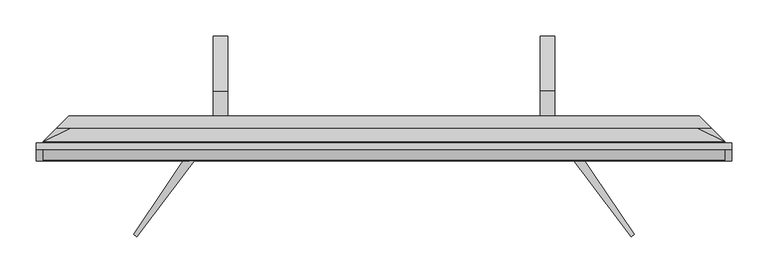
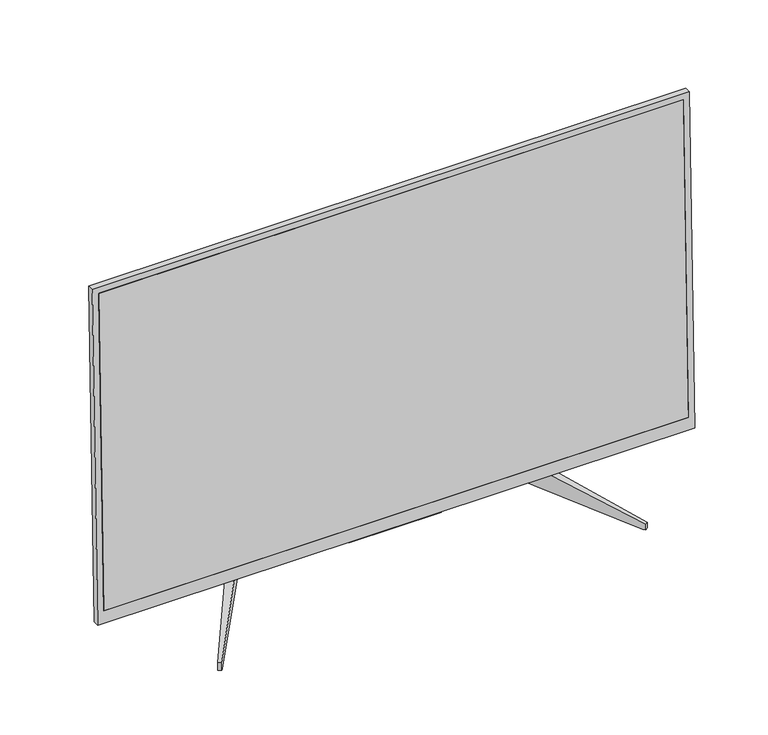
"""IFC4 building model written with IfcOpenShell, lengths in millimetres: proxy geometry, Electronics_Visual-TVs_Sony-Professional_FW-43BZ35F-43in-BRAVIA-4K-HDR-Professional-Display : FW-43BZ35F."""

from ifc_helpers import new_model, si_unit, point, frame, frame_2d, origin, place, context, project, spatial, polyline, circle_curve, trimmed, segment, composite_curve, outline, extrude, faceted_brep, source, transform, mapped, element, save
from ifc_brep_helpers import plane_surface, revolved_surface, advanced_brep


def communication_devices_8732f4fb(model_context):
    return source(origin(), model_context, "Body", "SolidModel", [
        extrude(outline(polyline([(0.0, -10.0000001), (0.0, 0.0), (944.8, 0.0), (944.8, -10.0000001), (0.0, -10.0000001)])), frame((472.4, -33.3449697, 83.2957538), z_axis=(0.0, 0.02617694830787593, 0.9996573249755573), x_axis=(-1.0, 0.0, 0.0)), (0.0, 0.0, 1.0), 534.3),
        faceted_brep([(482.4, -33.9, 62.1), (482.4, -23.8965721, 62.1), (482.4, -9.0936706, 627.4), (482.4, -19.0970985, 627.4), (-482.4, -33.9, 62.1), (-482.4, -19.0970985, 627.4), (-482.4, -9.0936706, 627.4), (-482.4, -23.8965721, 62.1), (-472.4, -23.3483964, 83.0339843), (472.4, -23.3483964, 83.0339843), (472.4, -9.3620529, 617.150893), (-472.4, -9.3620529, 617.150893), (472.4, -33.3449697, 83.2957538), (-472.4, -33.3449697, 83.2957538), (-472.4, -19.3586262, 617.4126625), (472.4, -19.3586262, 617.4126625)], [[[0, 1, 2, 3]], [[4, 5, 6, 7]], [[1, 0, 4, 7]], [[2, 1, 7, 6], [8, 9, 10, 11]], [[0, 3, 5, 4], [12, 13, 14, 15]], [[8, 13, 12, 9]], [[9, 12, 15, 10]], [[10, 15, 14, 11]], [[13, 8, 11, 14]], [[3, 2, 6, 5]]]),
        faceted_brep([(-236.5680468, 139.3, 32.6847301), (-216.5680468, 139.3, 32.6847301), (-216.5680468, 130.7, 0.0), (-236.5680468, 130.7, 0.0), (-216.5680468, 28.1, 37.1705579), (-236.5680468, 28.1, 37.1705579), (-236.5680468, 120.1003592, 0.0), (-216.5680468, 120.1003592, 0.0), (-236.5680468, 62.670602, 62.1), (-216.5680468, 62.670602, 62.1), (-339.9507568, -135.8671682, 0.0), (-347.1652982, -135.8671682, 0.0), (-216.5680468, 28.1, 62.1), (-236.5680468, 28.1, 62.1), (-258.0876491, -3.8041224, 62.1), (-246.471337, -11.6394239, 62.1), (-342.5339087, -139.3, 0.0), (-347.1652982, -135.8671682, 13.3980759), (-342.5339087, -139.3, 13.3197763)], [[[0, 1, 2, 3]], [[4, 5, 6, 7]], [[1, 0, 8, 9]], [[5, 4, 10, 11]], [[12, 9, 8, 13, 14, 15]], [[16, 11, 10]], [[6, 3, 2, 7]], [[13, 5, 11, 17, 14]], [[11, 16, 18, 17]], [[16, 10, 4, 12, 15, 18]], [[9, 12, 4, 7, 2, 1]], [[13, 8, 0, 3, 6, 5]], [[15, 14, 17, 18]]]),
        faceted_brep([(236.5680468, 28.1, 62.1), (236.5680468, 62.670602, 62.1), (216.5680468, 62.670602, 62.1), (216.5680468, 28.1, 62.1), (238.7109742, -1.3264334, 62.1), (250.8799901, 6.8816715, 62.1), (347.1652982, -135.8671682, 0.0), (342.5339087, -139.3, 0.0), (339.9507568, -135.8671682, 0.0), (216.5680468, 120.1003592, 0.0), (216.5680468, 130.7, 0.0), (236.5680468, 130.7, 0.0), (236.5680468, 120.1003592, 0.0), (236.5680468, 28.1, 37.1705579), (347.1652982, -135.8671682, 9.4573919), (342.5339087, -139.3, 9.3790923), (216.5680468, 28.1, 37.1705579), (216.5680468, 139.3, 32.6847301), (236.5680468, 139.3, 32.6847301)], [[[0, 1, 2, 3, 4, 5]], [[6, 7, 8]], [[9, 10, 11, 12]], [[13, 0, 5, 14, 6]], [[7, 6, 14, 15]], [[8, 7, 15, 4, 3, 16]], [[3, 2, 17, 10, 9, 16]], [[1, 0, 13, 12, 11, 18]], [[17, 18, 11, 10]], [[13, 16, 9, 12]], [[18, 17, 2, 1]], [[16, 13, 6, 8]], [[5, 4, 15, 14]]]),
        extrude(outline(composite_curve([segment(trimmed(circle_curve(frame_2d((64.9596066, 9.5619733)), 10.0), [point((64.9596066, 19.5619733))], [point((74.9596066, 9.5619733))], False, "CARTESIAN"), True, "CONTINUOUS"), segment(polyline([(74.9596066, 9.5619733), (74.9596066, -30.5494977), (-74.9596066, -30.5494977), (-74.9596066, 9.5619733)]), True, "CONTINUOUS"), segment(trimmed(circle_curve(frame_2d((-64.9596066, 9.5619733)), 10.0), [point((-74.9596066, 9.5619733))], [point((-64.9596066, 19.5619733))], False, "CARTESIAN"), True, "CONTINUOUS"), segment(polyline([(-64.9596066, 19.5619733), (64.9596066, 19.5619733)]), True, "CONTINUOUS")], self_intersect=False)), frame((0.0, 0.0, 58.1), z_axis=(0.0, 0.0, 1.0), x_axis=(1.0, 0.0, 0.0)), (0.0, 0.0, 1.0), 4.0),
        faceted_brep([(-472.4, -7.1375823, 617.1811048), (-472.4, -9.3612618, 617.1811048), (472.4, -9.3612618, 617.1811048), (472.4, -7.1375823, 617.1811048), (471.9010922, -6.8942487, 617.1811048), (-471.9010922, -6.8942487, 617.1811048), (435.1742293, 11.0186392, 526.6060744), (472.4, -7.1375823, 526.6060744), (472.4, -11.7330524, 526.6060744), (-472.4, -11.7330524, 526.6060744), (-472.4, -7.1375823, 526.6060744), (-435.1742293, 11.0186392, 526.6060744)], [[[0, 1, 2, 3, 4, 5]], [[6, 7, 8, 9, 10, 11]], [[0, 10, 9, 1]], [[7, 3, 2, 8]], [[2, 1, 9, 8]], [[11, 10, 0, 5]], [[7, 6, 4, 3]], [[5, 4, 6, 11]]]),
        advanced_brep(
        [(-472.4, -7.1375823, 526.6060744), (-472.4, -11.7330524, 526.6060744), (472.4, -11.7330524, 526.6060744), (472.4, -7.1375823, 526.6060744), (454.2437785, 11.0186392, 526.6060744), (-454.2437785, 11.0186392, 526.6060744), (-472.4, -7.1375823, 170.6631269), (-437.1624177, 28.1, 170.6631269), (437.1624177, 28.1, 170.6631269), (472.4, -7.1375823, 170.6631269), (472.4, -21.0537465, 170.6631269), (-472.4, -21.0537465, 170.6631269), (437.1624177, 28.1, 523.5941696), (-437.1624177, 28.1, 172.1), (-322.3011917, 28.1, 172.1), (-322.3011917, 28.1, 473.9795749), (-437.1624177, 28.1, 473.9795749), (-437.1624177, 28.1, 523.5941696), (212.1, 28.1, 266.75), (160.2, 28.1, 266.75), (160.2, 28.1, 179.75), (212.1, 28.1, 179.75), (-147.0, 28.1, 343.2), (-293.6, 28.1, 343.2), (-293.6, 28.1, 253.0), (-147.0, 28.1, 253.0), (100.0, 28.1, 326.3), (100.0, 28.1, 320.3), (-100.0, 28.1, 326.3), (-100.0, 28.1, 320.3), (-452.5963815, 12.6660362, 473.9795749), (-452.5963815, 12.6660362, 172.1), (-322.3011917, 12.6660362, 473.9795749), (-322.3011917, 12.6660362, 172.1), (212.1, 25.6497626, 266.75), (212.1, 25.6497626, 179.75), (160.2, 25.6497626, 179.75), (160.2, 25.6497626, 266.75), (-147.0, 25.6497626, 343.2), (-147.0, 25.6497626, 253.0), (-293.6, 25.6497626, 253.0), (-293.6, 25.6497626, 343.2), (100.0, 21.959368, 326.3), (100.0, 21.959368, 320.3), (-100.0, 21.959368, 326.3), (-100.0, 21.959368, 320.3)],
        [
            (0, 1),
            (1, 2),
            (2, 3),
            (3, 4),
            (4, 5),
            (5, 0),
            (6, 7),
            (7, 8),
            (8, 9),
            (9, 10),
            (10, 11),
            (11, 6),
            (0, 6),
            (11, 1),
            (9, 3),
            (2, 10),
            (8, 12),
            (12, 4),
            (7, 13),
            (13, 14),
            (14, 15),
            (15, 16),
            (16, 17),
            (17, 12),
            (18, 19),
            (19, 20),
            (20, 21),
            (21, 18),
            (22, 23),
            (23, 24),
            (24, 25),
            (25, 22),
            (26, 27, circle_curve(frame((100.0, 28.1, 323.3), z_axis=(0.0, -1.0, 0.0), x_axis=(0.0, 0.0, -1.0)), 3.0)),
            (27, 26, circle_curve(frame((100.0, 28.1, 323.3), z_axis=(0.0, -1.0, 0.0), x_axis=(0.0, 0.0, -1.0)), 3.0)),
            (28, 29, circle_curve(frame((-100.0, 28.1, 323.3), z_axis=(0.0, -1.0, 0.0), x_axis=(0.0, 0.0, -1.0)), 3.0)),
            (29, 28, circle_curve(frame((-100.0, 28.1, 323.3), z_axis=(0.0, -1.0, 0.0), x_axis=(0.0, 0.0, -1.0)), 3.0)),
            (5, 17),
            (16, 30),
            (30, 31),
            (31, 13),
            (32, 33),
            (33, 31),
            (30, 32),
            (32, 15),
            (14, 33),
            (34, 35),
            (35, 36),
            (36, 37),
            (37, 34),
            (38, 39),
            (39, 40),
            (40, 41),
            (41, 38),
            (37, 19),
            (18, 34),
            (36, 20),
            (35, 21),
            (41, 23),
            (22, 38),
            (40, 24),
            (39, 25),
            (42, 43, circle_curve(frame((100.0, 21.959368, 323.3), z_axis=(0.0, 1.0, 0.0), x_axis=(0.0, 0.0, -1.0)), 3.0)),
            (43, 42, circle_curve(frame((100.0, 21.959368, 323.3), z_axis=(0.0, 1.0, 0.0), x_axis=(0.0, 0.0, -1.0)), 3.0)),
            (44, 45, circle_curve(frame((-100.0, 21.959368, 323.3), z_axis=(0.0, 1.0, 0.0), x_axis=(0.0, 0.0, -1.0)), 3.0)),
            (45, 44, circle_curve(frame((-100.0, 21.959368, 323.3), z_axis=(0.0, 1.0, 0.0), x_axis=(0.0, 0.0, -1.0)), 3.0)),
            (43, 27),
            (26, 42),
            (45, 29),
            (28, 44),
        ],
        [
            plane_surface(frame((-472.4, -7.1375823, 526.6060744), z_axis=(0.0, 0.0, 1.0), x_axis=(0.0, -1.0, 0.0))),
            plane_surface(frame((-472.4, -7.1375823, 170.6631269), z_axis=(0.0, 0.0, -1.0), x_axis=(0.0, 1.0, 0.0))),
            plane_surface(frame((-472.4, -7.1375823, 526.6060744), z_axis=(-1.0, 0.0, 0.0), x_axis=(0.0, 0.0, -1.0))),
            plane_surface(frame((472.4, -27.5708403, 526.6060744), z_axis=(1.0, 0.0, 0.0), x_axis=(0.0, 0.0, -1.0))),
            plane_surface(frame((472.4, -7.1375823, 526.6060744), z_axis=(0.707106781186642, 0.7071067811864531, 0.0), x_axis=(0.0, 0.0, -1.0))),
            plane_surface(frame((437.1624177, 28.1, 526.6060744), z_axis=(0.0, 1.0, 0.0), x_axis=(0.0, 0.0, -1.0))),
            plane_surface(frame((-437.1624177, 28.1, 526.6060744), z_axis=(-0.7071067811865435, 0.7071067811865518, 0.0), x_axis=(0.0, 0.0, -1.0))),
            plane_surface(frame((625.5732366, -23.8965721, 62.1), z_axis=(0.0, -0.9996573249755574, 0.026176948307870252), x_axis=(-1.0, 0.0, 0.0))),
            plane_surface(frame((587.9862131, 11.0186392, 526.6060744), z_axis=(0.0, 0.17364817766693166, 0.9848077530122079), x_axis=(-1.0, 0.0, 0.0))),
            plane_surface(frame((-322.3011917, 12.6660362, 172.1), z_axis=(0.0, 1.0, 0.0), x_axis=(1.0, 0.0, 0.0))),
            plane_surface(frame((-322.3011917, 12.6660362, 172.1), z_axis=(-1.0, 0.0, 0.0), x_axis=(0.0, 1.0, 0.0))),
            plane_surface(frame((-322.3011917, 12.6660362, 473.9795749), z_axis=(0.0, 0.0, -1.0), x_axis=(0.0, 1.0, 0.0))),
            plane_surface(frame((-464.2088994, 12.6660362, 172.1), z_axis=(0.0, 0.0, 1.0), x_axis=(0.0, 1.0, 0.0))),
            plane_surface(frame((194.45, 25.6497626, 266.75), z_axis=(0.0, 1.0, 0.0), x_axis=(-1.0, 0.0, 0.0))),
            plane_surface(frame((212.1, 25.6497626, 266.75), z_axis=(0.0, 0.0, -1.0), x_axis=(0.0, 1.0, 0.0))),
            plane_surface(frame((160.2, 25.6497626, 266.75), z_axis=(1.0, 0.0, 0.0), x_axis=(0.0, 1.0, 0.0))),
            plane_surface(frame((160.2, 25.6497626, 179.75), z_axis=(0.0, 0.0, 1.0), x_axis=(0.0, 1.0, 0.0))),
            plane_surface(frame((212.1, 25.6497626, 179.75), z_axis=(-1.0, 0.0, 0.0), x_axis=(0.0, 1.0, 0.0))),
            plane_surface(frame((-147.0, 25.6497626, 343.2), z_axis=(0.0, 0.0, -1.0), x_axis=(0.0, 1.0, 0.0))),
            plane_surface(frame((-293.6, 25.6497626, 343.2), z_axis=(1.0, 0.0, 0.0), x_axis=(0.0, 1.0, 0.0))),
            plane_surface(frame((-293.6, 25.6497626, 253.0), z_axis=(0.0, 0.0, 1.0), x_axis=(0.0, 1.0, 0.0))),
            plane_surface(frame((-147.0, 25.6497626, 253.0), z_axis=(-1.0, 0.0, 0.0), x_axis=(0.0, 1.0, 0.0))),
            plane_surface(frame((100.0, 21.959368, 320.3), z_axis=(0.0, 1.0, 0.0), x_axis=(1.0, 0.0, 0.0))),
            revolved_surface(polyline([(100.0, 21.959368, 320.3), (100.0, 28.1, 320.3)]), (100.0, 36.8651248, 323.3), (0.0, -1.0, 0.0)),
            revolved_surface(polyline([(-100.0, 21.959368, 320.3), (-100.0, 28.1, 320.3)]), (-100.0, 36.8651248, 323.3), (0.0, -1.0, 0.0)),
        ],
        [
            (0, [[1, 2, 3, 4, 5, 6]]),
            (1, [[7, 8, 9, 10, 11, 12]]),
            (2, [[13, -12, 14, -1]]),
            (3, [[15, -3, 16, -10]]),
            (4, [[-9, 17, 18, -4, -15]]),
            (5, [[-8, 19, 20, 21, 22, 23, 24, -17], [25, 26, 27, 28], [29, 30, 31, 32], [33, 34], [35, 36]]),
            (6, [[-7, -13, -6, 37, -23, 38, 39, 40, -19]]),
            (7, [[-2, -14, -11, -16]]),
            (8, [[-5, -18, -24, -37]]),
            (9, [[41, 42, -39, 43]]),
            (10, [[-41, 44, -21, 45]]),
            (11, [[-43, -38, -22, -44]]),
            (12, [[-42, -45, -20, -40]]),
            (13, [[46, 47, 48, 49]]),
            (13, [[50, 51, 52, 53]]),
            (14, [[-49, 54, -25, 55]]),
            (15, [[-48, 56, -26, -54]]),
            (16, [[-47, 57, -27, -56]]),
            (17, [[-46, -55, -28, -57]]),
            (18, [[-53, 58, -29, 59]]),
            (19, [[-52, 60, -30, -58]]),
            (20, [[-51, 61, -31, -60]]),
            (21, [[-50, -59, -32, -61]]),
            (22, [[62, 63]]),
            (22, [[64, 65]]),
            (23, [[-63, 66, -33, 67]]),
            (23, [[-62, -67, -34, -66]]),
            (24, [[-65, 68, -35, 69]]),
            (24, [[-64, -69, -36, -68]]),
        ],
    ),
        advanced_brep(
        [(437.1624177, 28.1, 170.6631269), (-437.1624177, 28.1, 170.6631269), (-472.4, -7.1375823, 170.6631269), (-472.4, -21.0537465, 170.6631269), (472.4, -21.0537465, 170.6631269), (472.4, -7.1375823, 170.6631269), (437.1624177, 28.1, 62.1), (472.4, -7.1375823, 62.1), (472.4, -23.8965721, 62.1), (-472.4, -23.8965721, 62.1), (-472.4, -7.1375823, 62.1), (-437.1624177, 28.1, 62.1), (100.0, 28.1, 126.3), (100.0, 28.1, 120.3), (-100.0, 28.1, 126.3), (-100.0, 28.1, 120.3), (100.0, 21.959368, 126.3), (100.0, 21.959368, 120.3), (-100.0, 21.959368, 126.3), (-100.0, 21.959368, 120.3)],
        [
            (0, 1),
            (1, 2),
            (2, 3),
            (3, 4),
            (4, 5),
            (5, 0),
            (6, 7),
            (7, 8),
            (8, 9),
            (9, 10),
            (10, 11),
            (11, 6),
            (0, 6),
            (11, 1),
            (12, 13, circle_curve(frame((100.0, 28.1, 123.3), z_axis=(0.0, -1.0, 0.0), x_axis=(0.0, 0.0, -1.0)), 3.0)),
            (13, 12, circle_curve(frame((100.0, 28.1, 123.3), z_axis=(0.0, -1.0, 0.0), x_axis=(0.0, 0.0, -1.0)), 3.0)),
            (14, 15, circle_curve(frame((-100.0, 28.1, 123.3), z_axis=(0.0, -1.0, 0.0), x_axis=(0.0, 0.0, -1.0)), 3.0)),
            (15, 14, circle_curve(frame((-100.0, 28.1, 123.3), z_axis=(0.0, -1.0, 0.0), x_axis=(0.0, 0.0, -1.0)), 3.0)),
            (2, 10),
            (9, 3),
            (7, 5),
            (4, 8),
            (16, 17, circle_curve(frame((100.0, 21.959368, 123.3), z_axis=(0.0, 1.0, 0.0), x_axis=(0.0, 0.0, -1.0)), 3.0)),
            (17, 16, circle_curve(frame((100.0, 21.959368, 123.3), z_axis=(0.0, 1.0, 0.0), x_axis=(0.0, 0.0, -1.0)), 3.0)),
            (18, 19, circle_curve(frame((-100.0, 21.959368, 123.3), z_axis=(0.0, 1.0, 0.0), x_axis=(0.0, 0.0, -1.0)), 3.0)),
            (19, 18, circle_curve(frame((-100.0, 21.959368, 123.3), z_axis=(0.0, 1.0, 0.0), x_axis=(0.0, 0.0, -1.0)), 3.0)),
            (17, 13),
            (12, 16),
            (19, 15),
            (14, 18),
        ],
        [
            plane_surface(frame((-437.1624177, 28.1, 170.6631269), z_axis=(0.0, 0.0, 1.0), x_axis=(-1.0, 0.0, 0.0))),
            plane_surface(frame((-437.1624177, 28.1, 62.1), z_axis=(0.0, 0.0, -1.0), x_axis=(1.0, 0.0, 0.0))),
            plane_surface(frame((437.1624177, 28.1, 170.6631269), z_axis=(0.0, 1.0, 0.0), x_axis=(0.0, 0.0, -1.0))),
            plane_surface(frame((-472.4, -7.1375823, 170.6631269), z_axis=(-1.0, 0.0, 0.0), x_axis=(0.0, 0.0, -1.0))),
            plane_surface(frame((472.4, -27.5708403, 170.6631269), z_axis=(1.0, 0.0, 0.0), x_axis=(0.0, 0.0, -1.0))),
            plane_surface(frame((-437.1624177, 28.1, 170.6631269), z_axis=(-0.7071067811865488, 0.7071067811865462, 0.0), x_axis=(0.0, 0.0, -1.0))),
            plane_surface(frame((472.4, -7.1375823, 170.6631269), z_axis=(0.7071067811866403, 0.7071067811864549, 0.0), x_axis=(0.0, 0.0, -1.0))),
            plane_surface(frame((625.5732366, -23.8965721, 62.1), z_axis=(0.0, -0.9996573249755574, 0.026176948307870252), x_axis=(-1.0, 0.0, 0.0))),
            plane_surface(frame((100.0, 21.959368, 320.3), z_axis=(0.0, 1.0, 0.0), x_axis=(1.0, 0.0, 0.0))),
            revolved_surface(polyline([(100.0, 21.959368, 120.3), (100.0, 28.1, 120.3)]), (100.0, 36.8651248, 123.3), (0.0, -1.0, 0.0)),
            revolved_surface(polyline([(-100.0, 21.959368, 120.3), (-100.0, 28.1, 120.3)]), (-100.0, 36.8651248, 123.3), (0.0, -1.0, 0.0)),
        ],
        [
            (0, [[1, 2, 3, 4, 5, 6]]),
            (1, [[7, 8, 9, 10, 11, 12]]),
            (2, [[-1, 13, -12, 14], [15, 16], [17, 18]]),
            (3, [[19, -10, 20, -3]]),
            (4, [[21, -5, 22, -8]]),
            (5, [[-2, -14, -11, -19]]),
            (6, [[-6, -21, -7, -13]]),
            (7, [[-4, -20, -9, -22]]),
            (8, [[23, 24]]),
            (8, [[25, 26]]),
            (9, [[-24, 27, -15, 28]]),
            (9, [[-23, -28, -16, -27]]),
            (10, [[-26, 29, -17, 30]]),
            (10, [[-25, -30, -18, -29]]),
        ],
    ),
    ])


if __name__ == "__main__":
    model = new_model("IFC4")
    model_context = context("Model", 3, world=origin())
    ifc_project = project(units=[si_unit("LENGTHUNIT", "METRE", prefix="MILLI")], contexts=[model_context])
    site = spatial("IfcSite", under=ifc_project)
    building = spatial("IfcBuilding", under=site)
    placement = place(None, origin())
    communication_devices_shape = communication_devices_8732f4fb(model_context)
    element("IfcBuildingElementProxy", 1, Name="Electronics_Visual-TVs_Sony-Professional_FW-43BZ35F-43in-BRAVIA-4K-HDR-Professional-Display : FW-43BZ35F", ObjectType="Electronics_Visual-TVs_Sony-Professional_FW-43BZ35F-43in-BRAVIA-4K-HDR-Professional-Display : FW-43BZ35F", at=placement, inside=building, context=model_context, shape_type="MappedRepresentation", body=[
        mapped(communication_devices_shape, transform((0.0, 0.0, 0.0), x_axis=(1.0, 0.0, 0.0), y_axis=(0.0, 1.0, 0.0), z_axis=(0.0, 0.0, 1.0))),
    ])
    save(model, "model.ifc")

# Revit data of these elements
# Type "Electronics_Visual-TVs_Sony-Professional_FW-43BZ35F-43in-BRAVIA-4K-HDR-Professional-Display : FW-43BZ35F"
#   Wireless LAN = "Integrated"
#   Wide Mode = "Wide zoom/Normal/Full/Zoom/14:9"
#   Voltage AC = "DC 19.5V"
#   Video Signal = "4096 x 2160p (24, 60 Hz), 3840 x 2160p (24, 30, 60 Hz), 1080p (30, 60 Hz), 1080/24p, 1080i (60 Hz), 720p (30, 60 Hz), 720/24p, 480p, 480i"
#   Video Processing = "4K X-Reality PRO"
#   Vesa Mount Size = "4 x 7 7/8 inch"
#   USB Play = "MPEG1: MPEG1/MPEG2PS: MPEG2/MPEG2TS (HDV, AVCHD): MPEG2, AVC/MP4 (XAVCS): AVC, MPEG4, HEVC/AVI: Xvid, MotionJpeg/ASF (WMV): VC1/MOV: AVC, MPEG4, MotionJpeg/MKV: Xvid, AVC, MPEG4, VP8.HEVC/WEBM: VP8/3GPP: MPEG4, AVC/MP3/ASF (WMA)/WAV/MP4AAC/FLAC/JPEG"
#   URL = "https://pro.sony/ue_US/"
#   Speaker Position = "Down Firing"
#   Screen size = "43 in. (42.5 in.)"
#   Response Time = "5 ms"
#   Product url = "https://pro.sony/ue_US/products/pro-displays/fw-43bz35f"
#   Product data url = "https://www.bimobject.com/sonyprofessional/product/fw-43bz35f-display"
#   Package Carton = "42 1/4 x 27 3/8 x 5 7/8 inch"
#   Operation Time = "24/7"
#   OS = "Android 7.0 Nougat"
#   Multicast / IPTV = ""
#   Motionflow = "Motionflow XR 960 (Native 120Hz)"
#   Model = "FW-43BZ35F"
#   Miracast = "Yes"
#   Manufacturer URL = "https://pro.sony/ue_US/"
#   Manufacturer = "Sony Professional"
#   Dynamic Contrast Ratio = "400000"
#   Display Resolution = "QFHD"
#   Display Device = "LCD"
#   Dimming Type = "Frame Dimming"
#   Description = "This slim, energy-efficient FW-43BZ35F BRAVIA professional display combines bright, beautiful 4K HDR image quality with easy operation, flexible networking/control, and extensive integration options."
#   DLNA = "Home Network Client, Home Network Renderer"
#   Contrast Ratio = "1400"
#   Connector 9 = "Digital Audio Output"
#   Connector 8 = "Analog Audio Input"
#   Connector 7 = "HDMI Connection"
#   Connector 6 = "HDMI Connection"
#   Connector 5 = "HDMI Connection"
#   Connector 4 = "HDMI Connection"
#   Connector 3 = "Composite Video Input"
#   Connector 2 = "HDCP 2.2 (for HDMI 1/2/3/4)"
#   Connector 12 = "Ethernet Connection"
#   Connector 11 = "USB"
#   Connector 10 = "USB"
#   Connector 1 = "DC 19.5V"
#   Connection 15 = "USB"
#   Connection 14 = "Composite Video (Y/Pb/Pr) Input"
#   Connection 13 = "RS-232C Control"
#   Compatible with HDR = "Yes (HDR10, HLG)"
#   Backlight Type = "Edge LED"
#   Audio Power Output = "10W + 10W"
#   AC Power Input = "AC ADAPTER"
#   Width with Stand = 3' - 1.99213"
#   Width = 3' - 1.99213"
#   Weight Package Carton = 15.00 lbm
#   Weight Display with Stand = 11.30 lbm
#   Weight Display Only = 10.80 lbm
#   Screen Viewing Angle = 178.00°
#   Power Standby = 0.5 W
#   Power = 120 W
#   Height with Stand = 2' - 0.72441"
#   Height = 1' - 10.40157"
#   Depth with Stand = 0' - 10.98425"
#   Depth = 0' - 2.28346"
#   Default Elevation = 4' - 0"
#   Brightness Full = 505
#   Aspect Ratio = 1.77778
#   Wi-Fi direct = yes
#   Wi-Fi Certified = yes
#   Stand Yes/No [instance default] = yes
#   Sleep Timer = yes
#   Power Saving Mode / Back = yes
#   On/Off Timer = yes
#   On Screen Clock = yes
#   Light Sensor = yes
#   Google Cast = yes
#   Firmware Update = yes
#   Edition number = 1
#   Easy HTML5 Signage embedded = yes
#   Dynamic Backlight Control = yes
#   4:3 Default = yes
#   Screen Material = Screen - Sony - Black_Matt
#   Bezel Material = Plastic - Sony - Black_Matt
# Element 1 (IfcBuildingElementProxy, "Electronics_Visual-TVs_Sony-Professional_FW-43BZ35F-43in-BRAVIA-4K-HDR-Professional-Display : FW-43BZ35F")
#   Materials on its faces: "Plastic - Sony - Black_Matt", "Plastic - Sony - Gray_Matt", "Screen - Sony - Black_Matt"
# Materials
#   "Screen - Sony - Black_Matt": class "Generic", colour RGB 48 48 48, transparency 0, Manufacturer = "Sony", URL = "www.sony.com", Description = "Screen Black Matt by Sony", Cost = 0
#   "Plastic - Sony - Black_Matt": class "Plastic", colour RGB 30 30 30, transparency 0, Manufacturer = "Sony", URL = "www.sony.com", Description = "Black Matt Plastic by Sony", Cost = 0
#   "Plastic - Sony - Gray_Matt": class "Plastic", colour RGB 63 63 63, transparency 0, Manufacturer = "Sony", URL = "www.sony.com", Description = "Gray Matt Plastic by Sony", Cost = 0
